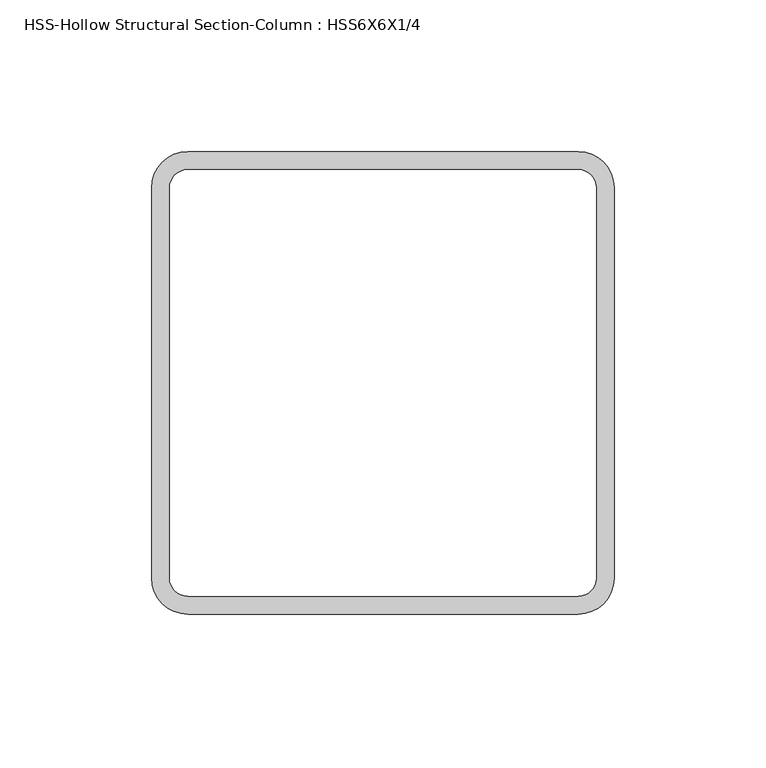
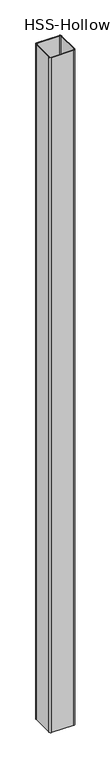
"""IFC4 building model written with IfcOpenShell, lengths in millimetres: column geometry, HSS-Hollow Structural Section-Column : HSS6X6X1/4."""

from ifc_helpers import new_model, si_unit, point, frame, frame_2d, origin, place, context, project, spatial, polyline, circle_curve, trimmed, segment, composite_curve, outline, extrude, source, transform, mapped, element, save


def hss_hollow_structural_section_column_hss6x6x1_4_ddf34e0a(model_context):
    return source(origin(), model_context, "Body", "SweptSolid", [
        extrude(outline(composite_curve([segment(trimmed(circle_curve(frame_2d((64.3636, 64.3636)), 11.8364), [point((64.3636, 76.2))], [point((76.2, 64.3636))], False, "CARTESIAN"), True, "CONTINUOUS"), segment(polyline([(76.2, 64.3636), (76.2, -64.3636)]), True, "CONTINUOUS"), segment(trimmed(circle_curve(frame_2d((64.3636, -64.3636)), 11.8364), [point((76.2, -64.3636))], [point((64.3636, -76.2))], False, "CARTESIAN"), True, "CONTINUOUS"), segment(polyline([(64.3636, -76.2), (-64.3636, -76.2)]), True, "CONTINUOUS"), segment(trimmed(circle_curve(frame_2d((-64.3636, -64.3636)), 11.8364), [point((-64.3636, -76.2))], [point((-76.2, -64.3636))], False, "CARTESIAN"), True, "CONTINUOUS"), segment(polyline([(-76.2, -64.3636), (-76.2, 64.3636)]), True, "CONTINUOUS"), segment(trimmed(circle_curve(frame_2d((-64.3636, 64.3636)), 11.8364), [point((-76.2, 64.3636))], [point((-64.3636, 76.2))], False, "CARTESIAN"), True, "CONTINUOUS"), segment(polyline([(-64.3636, 76.2), (64.3636, 76.2)]), True, "CONTINUOUS")], self_intersect=False), holes=[composite_curve([segment(polyline([(64.3636, 70.2818), (-64.3636, 70.2818)]), True, "CONTINUOUS"), segment(trimmed(circle_curve(frame_2d((-64.3636, 64.3636)), 5.9182), [point((-64.3636, 70.2818))], [point((-70.2818, 64.3636))], True, "CARTESIAN"), True, "CONTINUOUS"), segment(polyline([(-70.2818, 64.3636), (-70.2818, -64.3636)]), True, "CONTINUOUS"), segment(trimmed(circle_curve(frame_2d((-64.3636, -64.3636)), 5.9182), [point((-70.2818, -64.3636))], [point((-64.3636, -70.2818))], True, "CARTESIAN"), True, "CONTINUOUS"), segment(polyline([(-64.3636, -70.2818), (64.3636, -70.2818)]), True, "CONTINUOUS"), segment(trimmed(circle_curve(frame_2d((64.3636, -64.3636)), 5.9182), [point((64.3636, -70.2818))], [point((70.2818, -64.3636))], True, "CARTESIAN"), True, "CONTINUOUS"), segment(polyline([(70.2818, -64.3636), (70.2818, 64.3636)]), True, "CONTINUOUS"), segment(trimmed(circle_curve(frame_2d((64.3636, 64.3636)), 5.9182), [point((70.2818, 64.3636))], [point((64.3636, 70.2818))], True, "CARTESIAN"), True, "CONTINUOUS")], self_intersect=False)]), frame((0.0, 0.0, 27787.6), z_axis=(0.0, 0.0, 1.0), x_axis=(1.0, 0.0, 0.0)), (0.0, 0.0, 1.0), 4197.35),
    ])


if __name__ == "__main__":
    model = new_model("IFC4")
    model_context = context("Model", 3, world=origin())
    ifc_project = project(units=[si_unit("LENGTHUNIT", "METRE", prefix="MILLI")], contexts=[model_context])
    site = spatial("IfcSite", under=ifc_project)
    building = spatial("IfcBuilding", under=site)
    placement = place(None, origin())
    hss_hollow_structural_section_column_hss6x6x1_4_shape = hss_hollow_structural_section_column_hss6x6x1_4_ddf34e0a(model_context)
    element("IfcColumn", 1, ObjectType="HSS-Hollow Structural Section-Column : HSS6X6X1/4", at=placement, inside=building, context=model_context, shape_type="MappedRepresentation", body=[
        mapped(hss_hollow_structural_section_column_hss6x6x1_4_shape, transform((0.0, 0.0, 0.0), x_axis=(1.0, 0.0, 0.0), y_axis=(0.0, 1.0, 0.0), z_axis=(0.0, 0.0, 1.0))),
    ])
    save(model, "model.ifc")

# Revit data of these elements
# Type "HSS-Hollow Structural Section-Column : HSS6X6X1/4"
#   Assembly Code = "B10"
#   Shape = "Square"
#   W = 19
#   Ht = 0' - 6"
#   b = 0' - 6"
#   kr = 0' - 0.466"
#   t = 0' - 0.233"
#   A = 0.0363889 SF
#   Structural Material [instance default] = Steel ASTM A500, Grade B, Rectangular and Square
# Element 1 (IfcColumn, "HSS-Hollow Structural Section-Column : HSS6X6X1/4")
#   Materials on its faces: "Steel ASTM A500, Grade B, Rectangular and Square"
# Materials
#   "Steel ASTM A500, Grade B, Rectangular and Square": class "Metal", colour RGB 199 199 199, transparency 0, Description = "Carbon steel", Cost = 0
